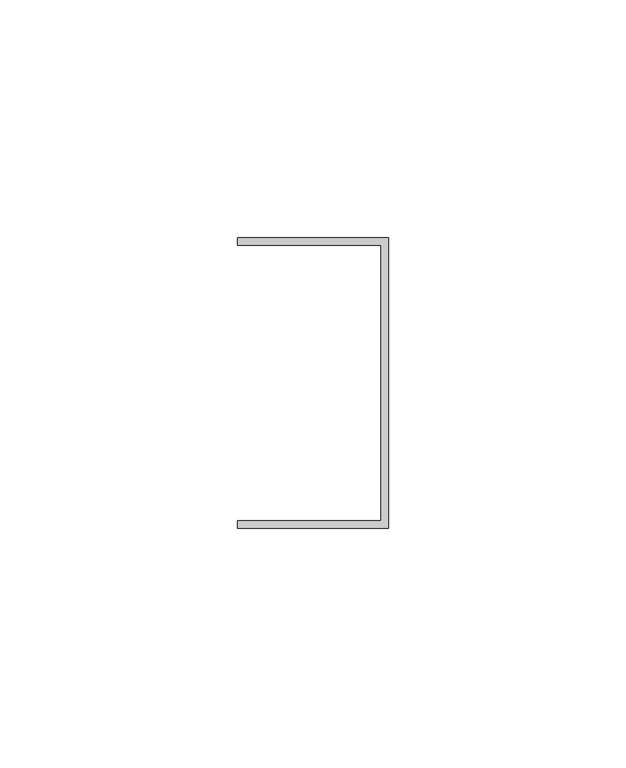
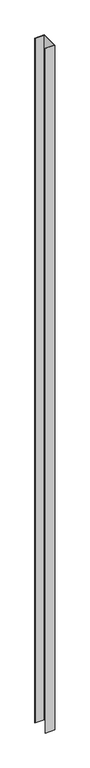
"""IFC4 building model written with IfcOpenShell, lengths in millimetres: proxy geometry, Generic Models 7:Generic Models 1:3:Generic Models 1:3 : Generic Models 7:Generic Models 1:305549:3:Generic Models 1:3:Generic Models 1:3 : Generic Models 7:Generic Models 1:305549:3 : Generic Models 7:Generic Models 1:3:Generic Models 1:3 : Generic Models 7:Generic Models 1:305549:301244:42 : Generic Models 7:Generic Models 1:3:Generic Models 1:3 : Generic Models 7:Generic Models 1:305549:3:Generic Models 1:3:Generic Models 1:3 : Generic Models 7:Generic Models 1:305549:3 : Generic Models 7:Generic Models 1:3:Generic Models 1:3 : Generic Models 7:Generic Models 1:305549:301244:308848."""

import ifcopenshell
import ifcopenshell.guid

model = None  # the IFC model being written
_history = None  # IfcOwnerHistory: only IFC2X3 demands one
_inside = {}  # id of a spatial element -> (the spatial element, [elements in it])
_under = {}  # id of a project, library or spatial element -> (it, [spatial elements below it])
_declared = {}  # id of a project -> (the project, [libraries it declares])
_typed = {}  # id of a type object -> (the type object, [elements of that type])
_made_of = {}  # id of a material, layer set ... -> (it, [elements and type objects made of it])


def new_model(schema):
    """Start an empty IFC model of exactly this schema.

    Asked for "IFC4X3", IfcOpenShell would pick the latest addendum, in which some entities
    have other attributes; the version numbers below select the first issue.
    IFC2X3 requires an IfcOwnerHistory on every rooted entity: one is made here for all.
    """
    global model, _history
    if schema == "IFC4X3":
        model = ifcopenshell.file(schema_version=(4, 3, 0, 0))
    else:
        model = ifcopenshell.file(schema=schema)
    _inside.clear()
    _under.clear()
    _declared.clear()
    _typed.clear()
    _made_of.clear()
    _history = None
    if model.schema == "IFC2X3":
        org = make("IfcOrganization", Name="unknown")
        user = make(
            "IfcPersonAndOrganization",
            ThePerson=make("IfcPerson", FamilyName="unknown"),
            TheOrganization=org,
        )
        app = make(
            "IfcApplication",
            ApplicationDeveloper=org,
            Version="unknown",
            ApplicationFullName="unknown",
            ApplicationIdentifier="unknown",
        )
        _history = make(
            "IfcOwnerHistory",
            OwningUser=user,
            OwningApplication=app,
            ChangeAction="ADDED",
            CreationDate=0,
        )
    return model


def make(cls, **values):
    """One entity of the class cls with the attributes given. An attribute that is None is left unset."""
    return model.create_entity(
        cls, **{name: value for name, value in values.items() if value is not None}
    )


def rooted(cls, **values):
    """An entity with a GlobalId (a new one), such as an element, a storey or a relation."""
    return make(cls, GlobalId=ifcopenshell.guid.new(), OwnerHistory=_history, **values)


def si_unit(unit_type, name, prefix=None):
    """IfcSIUnit, for example si_unit("LENGTHUNIT", "METRE", prefix="MILLI")."""
    return make("IfcSIUnit", UnitType=unit_type, Prefix=prefix, Name=name)


def assignment(units):
    """IfcUnitAssignment: the units of a project."""
    return None if units is None else make("IfcUnitAssignment", Units=units)


def point(xyz):
    """IfcCartesianPoint."""
    return None if xyz is None else make("IfcCartesianPoint", Coordinates=xyz)


def direction(xyz):
    """IfcDirection."""
    return None if xyz is None else make("IfcDirection", DirectionRatios=xyz)


def frame(location, z_axis=None, x_axis=None):
    """IfcAxis2Placement3D, a coordinate frame: its origin and axes. An axis left out is left unset."""
    return make(
        "IfcAxis2Placement3D",
        Location=point(location),
        Axis=direction(z_axis),
        RefDirection=direction(x_axis),
    )


def origin():
    """The frame at (0, 0, 0) with its axes left unset."""
    return frame((0.0, 0.0, 0.0))


def place(relative_to, where):
    """IfcLocalPlacement: puts the frame where relative to a parent placement (None: the world)."""
    return make(
        "IfcLocalPlacement", PlacementRelTo=relative_to, RelativePlacement=where
    )


def context(
    kind, dimensions, precision=None, world=None, true_north=None, identifier=None
):
    """IfcGeometricRepresentationContext, for example the 3D "Model" context."""
    return make(
        "IfcGeometricRepresentationContext",
        ContextIdentifier=identifier,
        ContextType=kind,
        CoordinateSpaceDimension=dimensions,
        Precision=precision,
        WorldCoordinateSystem=world,
        TrueNorth=true_north,
    )


def project(units=None, contexts=None):
    """IfcProject with its units and contexts."""
    return rooted(
        "IfcProject",
        Name="project",
        RepresentationContexts=contexts,
        UnitsInContext=assignment(units),
    )


def spatial(cls, under=None, at=None, **own):
    """A site, building, storey or space (cls), placed at a placement, below another one or the project."""
    s = rooted(cls, ObjectPlacement=at, **own)
    if under is not None:
        _under.setdefault(under.id(), (under, []))[1].append(s)
    return s


def polyline(points):
    """IfcPolyline through the points."""
    return make("IfcPolyline", Points=[point(p) for p in points])


def outline(outer, holes=None, kind="AREA"):
    """IfcArbitraryClosedProfileDef: a profile drawn as a closed curve; with holes, ...WithVoids."""
    if holes is None:
        return make("IfcArbitraryClosedProfileDef", ProfileType=kind, OuterCurve=outer)
    return make(
        "IfcArbitraryProfileDefWithVoids",
        ProfileType=kind,
        OuterCurve=outer,
        InnerCurves=holes,
    )


def extrude(swept, where, along, depth):
    """IfcExtrudedAreaSolid: the profile swept, set in the frame where, extruded along a direction by depth."""
    return make(
        "IfcExtrudedAreaSolid",
        SweptArea=swept,
        Position=where,
        ExtrudedDirection=direction(along),
        Depth=depth,
    )


def shape(context_of_items, identifier, shape_type, items):
    """IfcShapeRepresentation: the items that make up one representation, for example the "Body"."""
    return make(
        "IfcShapeRepresentation",
        ContextOfItems=context_of_items,
        RepresentationIdentifier=identifier,
        RepresentationType=shape_type,
        Items=items,
    )


def source(mapping_origin, context_of_items, identifier, shape_type, items):
    """IfcRepresentationMap: a shape defined once, which mapped items show again and again."""
    return make(
        "IfcRepresentationMap",
        MappingOrigin=mapping_origin,
        MappedRepresentation=shape(context_of_items, identifier, shape_type, items),
    )


def transform(
    local_origin,
    x_axis=None,
    y_axis=None,
    z_axis=None,
    scale=None,
    scale2=None,
    scale3=None,
    uniform=True,
):
    """IfcCartesianTransformationOperator3D, or its non-uniform kind. x_axis, y_axis, z_axis: its Axis1, 2, 3."""
    if uniform:
        return make(
            "IfcCartesianTransformationOperator3D",
            Axis1=direction(x_axis),
            Axis2=direction(y_axis),
            LocalOrigin=point(local_origin),
            Scale=scale,
            Axis3=direction(z_axis),
        )
    return make(
        "IfcCartesianTransformationOperator3DnonUniform",
        Axis1=direction(x_axis),
        Axis2=direction(y_axis),
        LocalOrigin=point(local_origin),
        Scale=scale,
        Axis3=direction(z_axis),
        Scale2=scale2,
        Scale3=scale3,
    )


def mapped(mapping_source, mapping_target):
    """IfcMappedItem: shows the shape of a source again, moved by a transform."""
    return make(
        "IfcMappedItem", MappingSource=mapping_source, MappingTarget=mapping_target
    )


def made_of(thing, what):
    """Note that an element or type object is made of a material, layer set ...; save() writes the relation."""
    if what is not None:
        _made_of.setdefault(what.id(), (what, []))[1].append(thing)
    return thing


def element(
    cls,
    number,
    at=None,
    inside=None,
    cuts=None,
    type_object=None,
    material=None,
    context=None,
    identifier="Body",
    shape_type=None,
    held_by="IfcProductDefinitionShape",
    body=None,
    shapes=None,
    **own,
):
    """One element of the class cls, such as IfcWall. Its Tag is "e" and its number.

    at: its placement. inside: the storey or other place that contains it. cuts: it is an
    opening in that element (IfcRelVoidsElement). A single representation is given by context,
    identifier, shape_type and body (its items); several are given by shapes. held_by: the class
    of the entity that holds the representations. save() writes the other relations.
    """
    e = rooted(cls, Tag="e%d" % number, ObjectPlacement=at, **own)
    if body is not None:
        shapes = [shape(context, identifier, shape_type, body)]
    if shapes is not None:
        e.Representation = make(held_by, Representations=shapes)
    if inside is not None:
        _inside.setdefault(inside.id(), (inside, []))[1].append(e)
    if cuts is not None:
        rooted(
            "IfcRelVoidsElement", RelatingBuildingElement=cuts, RelatedOpeningElement=e
        )
    if type_object is not None:
        _typed.setdefault(type_object.id(), (type_object, []))[1].append(e)
    return made_of(e, material)


def aggregate(whole, parts):
    """IfcRelAggregates: a whole, such as a stair, and the parts it consists of."""
    return rooted("IfcRelAggregates", RelatingObject=whole, RelatedObjects=parts)


def save(model, path):
    """Write the relations noted so far, then the file.

    IfcRelAggregates (storeys below a building ...), IfcRelContainedInSpatialStructure (elements
    in a storey), IfcRelDefinesByType, IfcRelAssociatesMaterial and IfcRelDeclares: one each for
    every whole, place, type object, material and project.
    """
    for whole, parts in _under.values():
        aggregate(whole, parts)
    for where, things in _inside.values():
        rooted(
            "IfcRelContainedInSpatialStructure",
            RelatedElements=things,
            RelatingStructure=where,
        )
    for kind, things in _typed.values():
        rooted("IfcRelDefinesByType", RelatedObjects=things, RelatingType=kind)
    for what, things in _made_of.values():
        rooted("IfcRelAssociatesMaterial", RelatedObjects=things, RelatingMaterial=what)
    for by, libraries in _declared.values():
        rooted("IfcRelDeclares", RelatingContext=by, RelatedDefinitions=libraries)
    model.write(path)


def generic_models_4d4d2faa(model_context):
    return source(origin(), model_context, "Body", "SweptSolid", [
        extrude(outline(polyline([(560686.336724, -579015.772634), (560686.336724, -579076.8913841), (560654.586724, -579076.8913841), (560654.586724, -579075.3038841), (560684.749224, -579075.3038841), (560684.749224, -579017.360134), (560654.586724, -579017.360134), (560654.586724, -579015.772634), (560686.336724, -579015.772634)])), frame((0.0, 0.0, 3721.1), z_axis=(0.0, 0.0, 1.0), x_axis=(1.0, 0.0, 0.0)), (0.0, 0.0, 1.0), 2430.9324376),
    ])


if __name__ == "__main__":
    model = new_model("IFC4")
    model_context = context("Model", 3, world=origin())
    ifc_project = project(units=[si_unit("LENGTHUNIT", "METRE", prefix="MILLI")], contexts=[model_context])
    site = spatial("IfcSite", under=ifc_project)
    building = spatial("IfcBuilding", under=site)
    placement = place(None, origin())
    generic_models_shape = generic_models_4d4d2faa(model_context)
    element("IfcBuildingElementProxy", 1, Name="Generic Models 7:Generic Models 1:3:Generic Models 1:3 : Generic Models 7:Generic Models 1:305549:3:Generic Models 1:3:Generic Models 1:3 : Generic Models 7:Generic Models 1:305549:3 : Generic Models 7:Generic Models 1:3:Generic Models 1:3 : Generic Models 7:Generic Models 1:305549:301244:42 : Generic Models 7:Generic Models 1:3:Generic Models 1:3 : Generic Models 7:Generic Models 1:305549:3:Generic Models 1:3:Generic Models 1:3 : Generic Models 7:Generic Models 1:305549:3 : Generic Models 7:Generic Models 1:3:Generic Models 1:3 : Generic Models 7:Generic Models 1:305549:301244:308848", ObjectType="Generic Models 7:Generic Models 1:3:Generic Models 1:3 : Generic Models 7:Generic Models 1:305549:3:Generic Models 1:3:Generic Models 1:3 : Generic Models 7:Generic Models 1:305549:3 : Generic Models 7:Generic Models 1:3:Generic Models 1:3 : Generic Models 7:Generic Models 1:305549:301244:42 : Generic Models 7:Generic Models 1:3:Generic Models 1:3 : Generic Models 7:Generic Models 1:305549:3:Generic Models 1:3:Generic Models 1:3 : Generic Models 7:Generic Models 1:305549:3 : Generic Models 7:Generic Models 1:3:Generic Models 1:3 : Generic Models 7:Generic Models 1:305549:301244:308848", at=placement, inside=building, context=model_context, shape_type="MappedRepresentation", body=[
        mapped(generic_models_shape, transform((0.0, 0.0, 0.0), x_axis=(1.0, 0.0, 0.0), y_axis=(0.0, 1.0, 0.0), z_axis=(0.0, 0.0, 1.0))),
    ])
    save(model, "model.ifc")

# Revit data of these elements
# Type "Generic Models 7:Generic Models 1:3:Generic Models 1:3 : Generic Models 7:Generic Models 1:305549:3:Generic Models 1:3:Generic Models 1:3 : Generic Models 7:Generic Models 1:305549:3 : Generic Models 7:Generic Models 1:3:Generic Models 1:3 : Generic Models 7:Generic Models 1:305549:301244:42 : Generic Models 7:Generic Models 1:3:Generic Models 1:3 : Generic Models 7:Generic Models 1:305549:3:Generic Models 1:3:Generic Models 1:3 : Generic Models 7:Generic Models 1:305549:3 : Generic Models 7:Generic Models 1:3:Generic Models 1:3 : Generic Models 7:Generic Models 1:305549:301244:308848"
#   NameOverride = "Generic Models 7:Generic Models 1:3:Generic Models 1:3 : Generic Models 7:Generic Models 1:305549:3:Generic Models 1:3:Generic Models 1:3 : Generic Models 7:Generic Models 1:305549:3 : Generic Models 7:Generic Models 1:3:Generic Models 1:3 : Generic Models 7:Generic Models 1:305549:301244:308848"
#   ObjectTypeOverride = "Generic Models 1:3:Generic Models 1:3 : Generic Models 7:Generic Models 1:305549:3 : Generic Models 7:Generic Models 1:3:Generic Models 1:3 : Generic Models 7:Generic Models 1:305549:301244"
#   Reference = "Generic Models 1"
#   Tag = "308848"
# Element 1 (IfcBuildingElementProxy, "Generic Models 7:Generic Models 1:3:Generic Models 1:3 : Generic Models 7:Generic Models 1:305549:3:Generic Models 1:3:Generic Models 1:3 : Generic Models 7:Generic Models 1:305549:3 : Generic Models 7:Generic Models 1:3:Generic Models 1:3 : Generic Models 7:Generic Models 1:305549:301244:42 : Generic Models 7:Generic Models 1:3:Generic Models 1:3 : Generic Models 7:Generic Models 1:305549:3:Generic Models 1:3:Generic Models 1:3 : Generic Models 7:Generic Models 1:305549:3 : Generic Models 7:Generic Models 1:3:Generic Models 1:3 : Generic Models 7:Generic Models 1:305549:301244:308848")
#   Materials on its faces: "GALVANIZED U-CHANNEL (250T125-33)"
# Materials
#   "GALVANIZED U-CHANNEL (250T125-33)": class "Unassigned", colour RGB 202 201 200, transparency 0, Keynote = "M05451300.02", Cost = 0
